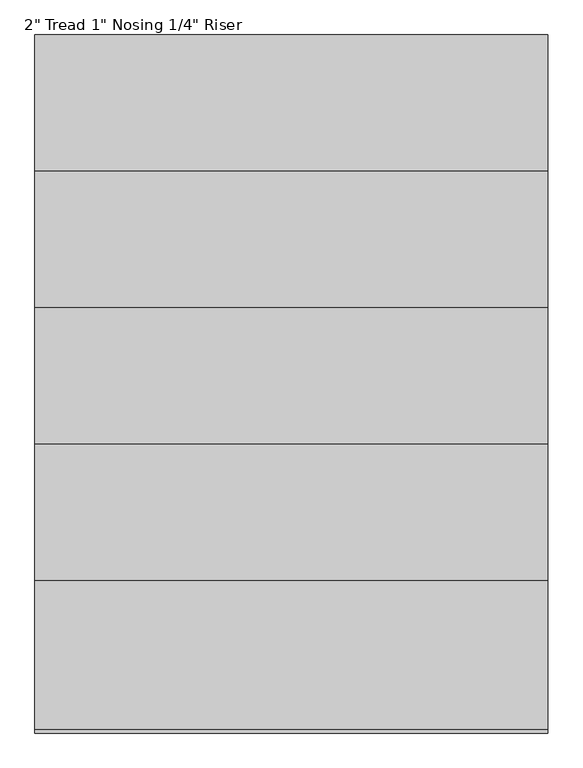
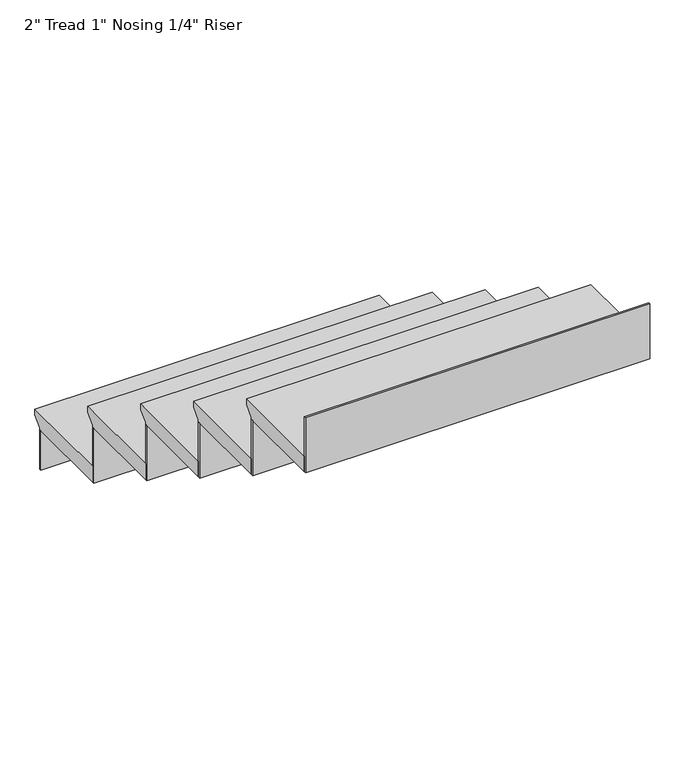
"""IFC4 building model written with IfcOpenShell, lengths in millimetres: stair flight geometry."""

from ifc_helpers import new_model, si_unit, frame, origin, place, context, project, spatial, polyline, outline, extrude, source, transform, mapped, element, save


def stair_flight_e0586406(model_context):
    return source(origin(), model_context, "Body", "SweptSolid", [
        extrude(outline(polyline([(16835.0111033, -889.0), (17139.8111033, -889.0), (17139.8111033, -908.05), (17114.4111033, -933.45), (17114.4111033, -939.8), (16835.0111033, -939.8), (16835.0111033, -889.0)])), frame((-1604.9625, 0.0, 0.0), z_axis=(1.0, 0.0, 0.0), x_axis=(0.0, 1.0, 0.0)), (0.0, 0.0, 1.0), 1049.6366598),
        extrude(outline(polyline([(-1604.9625, 17108.0611033), (-1604.9625, 17114.4111033), (-555.3258402, 17114.4111033), (-555.3258402, 17108.0611033), (-1604.9625, 17108.0611033)])), frame((0.0, 0.0, -1066.8), z_axis=(0.0, 0.0, 1.0), x_axis=(1.0, 0.0, 0.0)), (0.0, 0.0, 1.0), 127.0),
        extrude(outline(polyline([(-1604.9625, 16828.6611033), (-1604.9625, 16835.0111033), (-555.3258402, 16835.0111033), (-555.3258402, 16828.6611033), (-1604.9625, 16828.6611033)])), frame((0.0, 0.0, -939.8), z_axis=(0.0, 0.0, 1.0), x_axis=(1.0, 0.0, 0.0)), (0.0, 0.0, 1.0), 177.8),
        extrude(outline(polyline([(16555.6111033, -711.2), (16860.4111033, -711.2), (16860.4111033, -730.25), (16835.0111033, -755.65), (16835.0111033, -762.0), (16555.6111033, -762.0), (16555.6111033, -711.2)])), frame((-1604.9625, 0.0, 0.0), z_axis=(1.0, 0.0, 0.0), x_axis=(0.0, 1.0, 0.0)), (0.0, 0.0, 1.0), 1049.6366598),
        extrude(outline(polyline([(-1604.9625, 16549.2611033), (-1604.9625, 16555.6111033), (-555.3258402, 16555.6111033), (-555.3258402, 16549.2611033), (-1604.9625, 16549.2611033)])), frame((0.0, 0.0, -762.0), z_axis=(0.0, 0.0, 1.0), x_axis=(1.0, 0.0, 0.0)), (0.0, 0.0, 1.0), 177.8),
        extrude(outline(polyline([(16276.2111033, -533.4), (16581.0111033, -533.4), (16581.0111033, -552.45), (16555.6111033, -577.85), (16555.6111033, -584.2), (16276.2111033, -584.2), (16276.2111033, -533.4)])), frame((-1604.9625, 0.0, 0.0), z_axis=(1.0, 0.0, 0.0), x_axis=(0.0, 1.0, 0.0)), (0.0, 0.0, 1.0), 1049.6366598),
        extrude(outline(polyline([(-1604.9625, 16269.8611033), (-1604.9625, 16276.2111033), (-555.3258402, 16276.2111033), (-555.3258402, 16269.8611033), (-1604.9625, 16269.8611033)])), frame((0.0, 0.0, -584.2), z_axis=(0.0, 0.0, 1.0), x_axis=(1.0, 0.0, 0.0)), (0.0, 0.0, 1.0), 177.8),
        extrude(outline(polyline([(15996.8111033, -355.6), (16301.6111033, -355.6), (16301.6111033, -374.65), (16276.2111033, -400.05), (16276.2111033, -406.4), (15996.8111033, -406.4), (15996.8111033, -355.6)])), frame((-1604.9625, 0.0, 0.0), z_axis=(1.0, 0.0, 0.0), x_axis=(0.0, 1.0, 0.0)), (0.0, 0.0, 1.0), 1049.6366598),
        extrude(outline(polyline([(-1604.9625, 15990.4611033), (-1604.9625, 15996.8111033), (-555.3258402, 15996.8111033), (-555.3258402, 15990.4611033), (-1604.9625, 15990.4611033)])), frame((0.0, 0.0, -406.4), z_axis=(0.0, 0.0, 1.0), x_axis=(1.0, 0.0, 0.0)), (0.0, 0.0, 1.0), 177.8),
        extrude(outline(polyline([(15717.4111033, -177.8), (16022.2111033, -177.8), (16022.2111033, -196.85), (15996.8111033, -222.25), (15996.8111033, -228.6), (15717.4111033, -228.6), (15717.4111033, -177.8)])), frame((-1604.9625, 0.0, 0.0), z_axis=(1.0, 0.0, 0.0), x_axis=(0.0, 1.0, 0.0)), (0.0, 0.0, 1.0), 1049.6366598),
        extrude(outline(polyline([(-1604.9625, 15711.0611033), (-1604.9625, 15717.4111033), (-555.3258402, 15717.4111033), (-555.3258402, 15711.0611033), (-1604.9625, 15711.0611033)])), frame((0.0, 0.0, -228.6), z_axis=(0.0, 0.0, 1.0), x_axis=(1.0, 0.0, 0.0)), (0.0, 0.0, 1.0), 177.8),
    ])


if __name__ == "__main__":
    model = new_model("IFC4")
    model_context = context("Model", 3, world=origin())
    ifc_project = project(units=[si_unit("LENGTHUNIT", "METRE", prefix="MILLI")], contexts=[model_context])
    site = spatial("IfcSite", under=ifc_project)
    building = spatial("IfcBuilding", under=site)
    placement = place(None, origin())
    stair_flight_shape = stair_flight_e0586406(model_context)
    element("IfcStairFlight", 1, ObjectType="2\" Tread 1\" Nosing 1/4\" Riser", at=placement, inside=building, context=model_context, shape_type="MappedRepresentation", body=[
        mapped(stair_flight_shape, transform((0.0, 0.0, 0.0), x_axis=(1.0, 0.0, 0.0), y_axis=(0.0, 1.0, 0.0), z_axis=(0.0, 0.0, 1.0))),
    ])
    save(model, "model.ifc")
